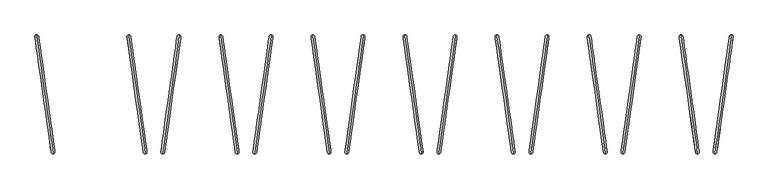
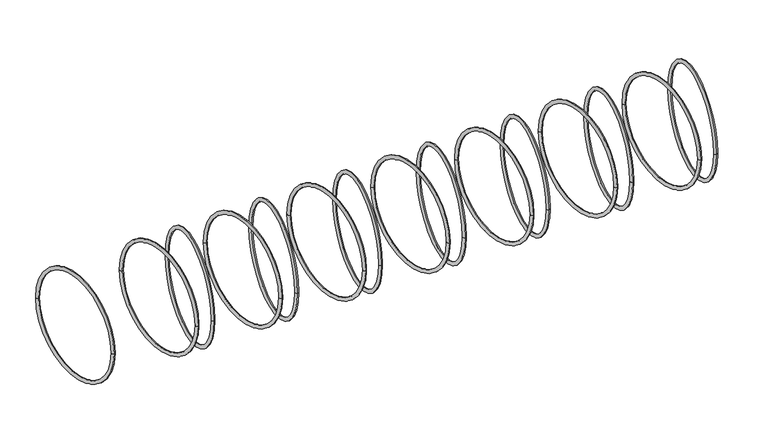
"""IFC4 building model written with IfcOpenShell, lengths in millimetres: geographic element geometry, NLRS_90_SI_WPB_fietsenrek staal_gen_bf : fietsenrek 5500mm 14 plaatsen."""

from ifc_helpers import new_model, si_unit, point, frame, origin, place, context, project, spatial, circle_curve, ellipse_curve, trimmed, source, transform, mapped, element, save
from ifc_brep_helpers import revolved_surface, advanced_brep


def geographic_element_fc57ddb0(model_context):
    return source(origin(), model_context, "Body", "AdvancedBrep", [
        advanced_brep(
        [(2160.5888305, 21.9255981, 304.7993564), (2162.7982034, 6.2050925, 304.7993564), (2089.8888952, 524.981777, 304.7993564), (2092.0982681, 509.2612714, 304.7993564)],
        [
            (0, 1, circle_curve(frame((2161.6935169, 14.0653453, 304.7993564), z_axis=(0.0, 0.0, 1.0), x_axis=(-0.1391731009600606, 0.990268068741571, 0.0)), 7.9375)),
            (1, 2, circle_curve(frame((2126.3435493, 265.5934347, 304.7993564), z_axis=(-0.990268068741571, -0.13917310096006058, 0.0), x_axis=(-0.13917310096006058, 0.990268068741571, 0.0)), 261.9375)),
            (2, 3, circle_curve(frame((2090.9935817, 517.1215242, 304.7993564), z_axis=(0.0, 0.0, 1.0), x_axis=(0.13917310096006055, -0.990268068741571, 0.0)), 7.9375)),
            (3, 0, circle_curve(frame((2126.3435493, 265.5934347, 304.7993564), z_axis=(0.990268068741571, 0.13917310096006058, 0.0), x_axis=(-0.13917310096006058, 0.990268068741571, 0.0)), 246.0625)),
            (1, 0, circle_curve(frame((2161.6935169, 14.0653453, 304.7993564), z_axis=(0.0, 0.0, 1.0), x_axis=(-0.1391731009600606, 0.990268068741571, 0.0)), 7.9375)),
            (3, 2, circle_curve(frame((2090.9935817, 517.1215242, 304.7993564), z_axis=(0.0, 0.0, 1.0), x_axis=(0.13917310096006055, -0.990268068741571, 0.0)), 7.9375)),
            (2, 1, circle_curve(frame((2126.3435493, 265.5934347, 304.7993564), z_axis=(-0.990268068741571, -0.13917310096006058, 0.0), x_axis=(0.13917310096006058, -0.990268068741571, 0.0)), 261.9375)),
            (0, 3, circle_curve(frame((2126.3435493, 265.5934347, 304.7993564), z_axis=(0.990268068741571, 0.13917310096006058, 0.0), x_axis=(0.13917310096006058, -0.990268068741571, 0.0)), 246.0625)),
        ],
        [
            revolved_surface(trimmed(ellipse_curve(frame((2090.9935817, 517.1215242, 304.7993564), z_axis=(0.0, 0.0, 1.0), x_axis=(0.13917310096006055, -0.990268068741571, 0.0)), 7.9375, 7.9375), [point((2089.8888952, 524.981777, 304.7993564))], [point((2092.0982681, 509.2612714, 304.7993564))], True, "CARTESIAN"), (2314.9896164, 292.1059105, 304.7993564), (-0.990268068741571, -0.13917310096006058, 0.0)),
            revolved_surface(trimmed(ellipse_curve(frame((2090.9935817, 517.1215242, 304.7993564), z_axis=(0.0, 0.0, 1.0), x_axis=(0.13917310096006055, -0.990268068741571, 0.0)), 7.9375, 7.9375), [point((2092.0982681, 509.2612714, 304.7993564))], [point((2089.8888952, 524.981777, 304.7993564))], True, "CARTESIAN"), (2314.9896164, 292.1059105, 304.7993564), (-0.990268068741571, -0.13917310096006058, 0.0)),
            revolved_surface(trimmed(ellipse_curve(frame((2161.6935169, 14.0653453, 304.7993564), z_axis=(0.0, 0.0, -1.0), x_axis=(-0.13917310096006055, 0.990268068741571, 0.0)), 7.9375, 7.9375), [point((2162.7982034, 6.2050925, 304.7993564))], [point((2160.5888305, 21.9255981, 304.7993564))], True, "CARTESIAN"), (2314.9896164, 292.1059105, 304.7993564), (-0.990268068741571, -0.13917310096006058, 0.0)),
            revolved_surface(trimmed(ellipse_curve(frame((2161.6935169, 14.0653453, 304.7993564), z_axis=(0.0, 0.0, -1.0), x_axis=(-0.13917310096006055, 0.990268068741571, 0.0)), 7.9375, 7.9375), [point((2160.5888305, 21.9255981, 304.7993564))], [point((2162.7982034, 6.2050925, 304.7993564))], True, "CARTESIAN"), (2314.9896164, 292.1059105, 304.7993564), (-0.990268068741571, -0.13917310096006058, 0.0)),
        ],
        [
            (0, [[1, 2, 3, 4]]),
            (1, [[5, -4, 6, -2]]),
            (2, [[-3, 7, -1, 8]]),
            (3, [[-6, -8, -5, -7]]),
        ],
    ),
        advanced_brep(
        [(2239.4111695, 21.9255981, 304.7993564), (2237.2017966, 6.2050925, 304.7993564), (2310.1111048, 524.981777, 304.7993564), (2307.9017319, 509.2612714, 304.7993564)],
        [
            (0, 1, circle_curve(frame((2238.3064831, 14.0653453, 304.7993564), z_axis=(0.0, 0.0, 1.0), x_axis=(0.13917310096005764, 0.9902680687415715, 0.0)), 7.9375)),
            (1, 2, circle_curve(frame((2273.6564507, 265.5934347, 304.7993564), z_axis=(-0.9902680687415715, 0.1391731009600577, 0.0), x_axis=(0.1391731009600577, 0.9902680687415715, 0.0)), 261.9375)),
            (2, 3, circle_curve(frame((2309.0064183, 517.1215242, 304.7993564), z_axis=(0.0, 0.0, 1.0), x_axis=(-0.13917310096005775, -0.9902680687415715, 0.0)), 7.9375)),
            (3, 0, circle_curve(frame((2273.6564507, 265.5934347, 304.7993564), z_axis=(0.9902680687415715, -0.1391731009600577, 0.0), x_axis=(0.1391731009600577, 0.9902680687415715, 0.0)), 246.0625)),
            (1, 0, circle_curve(frame((2238.3064831, 14.0653453, 304.7993564), z_axis=(0.0, 0.0, 1.0), x_axis=(0.13917310096005764, 0.9902680687415715, 0.0)), 7.9375)),
            (3, 2, circle_curve(frame((2309.0064183, 517.1215242, 304.7993564), z_axis=(0.0, 0.0, 1.0), x_axis=(-0.13917310096005775, -0.9902680687415715, 0.0)), 7.9375)),
            (2, 1, circle_curve(frame((2273.6564507, 265.5934347, 304.7993564), z_axis=(-0.9902680687415715, 0.1391731009600577, 0.0), x_axis=(-0.1391731009600577, -0.9902680687415715, 0.0)), 261.9375)),
            (0, 3, circle_curve(frame((2273.6564507, 265.5934347, 304.7993564), z_axis=(0.9902680687415715, -0.1391731009600577, 0.0), x_axis=(-0.1391731009600577, -0.9902680687415715, 0.0)), 246.0625)),
        ],
        [
            revolved_surface(trimmed(ellipse_curve(frame((2309.0064183, 517.1215242, 304.7993564), z_axis=(0.0, 0.0, 1.0), x_axis=(-0.13917310096005775, -0.9902680687415715, 0.0)), 7.9375, 7.9375), [point((2310.1111048, 524.981777, 304.7993564))], [point((2307.9017319, 509.2612714, 304.7993564))], True, "CARTESIAN"), (2085.0103836, 292.1059105, 304.7993564), (-0.9902680687415715, 0.1391731009600577, 0.0)),
            revolved_surface(trimmed(ellipse_curve(frame((2309.0064183, 517.1215242, 304.7993564), z_axis=(0.0, 0.0, 1.0), x_axis=(-0.13917310096005775, -0.9902680687415715, 0.0)), 7.9375, 7.9375), [point((2307.9017319, 509.2612714, 304.7993564))], [point((2310.1111048, 524.981777, 304.7993564))], True, "CARTESIAN"), (2085.0103836, 292.1059105, 304.7993564), (-0.9902680687415715, 0.1391731009600577, 0.0)),
            revolved_surface(trimmed(ellipse_curve(frame((2238.3064831, 14.0653453, 304.7993564), z_axis=(0.0, 0.0, -1.0), x_axis=(0.1391731009600577, 0.9902680687415715, 0.0)), 7.9375, 7.9375), [point((2237.2017966, 6.2050925, 304.7993564))], [point((2239.4111695, 21.9255981, 304.7993564))], True, "CARTESIAN"), (2085.0103836, 292.1059105, 304.7993564), (-0.9902680687415715, 0.1391731009600577, 0.0)),
            revolved_surface(trimmed(ellipse_curve(frame((2238.3064831, 14.0653453, 304.7993564), z_axis=(0.0, 0.0, -1.0), x_axis=(0.1391731009600577, 0.9902680687415715, 0.0)), 7.9375, 7.9375), [point((2239.4111695, 21.9255981, 304.7993564))], [point((2237.2017966, 6.2050925, 304.7993564))], True, "CARTESIAN"), (2085.0103836, 292.1059105, 304.7993564), (-0.9902680687415715, 0.1391731009600577, 0.0)),
        ],
        [
            (0, [[1, 2, 3, 4]]),
            (1, [[5, -4, 6, -2]]),
            (2, [[-3, 7, -1, 8]]),
            (3, [[-6, -8, -5, -7]]),
        ],
    ),
        advanced_brep(
        [(1760.5888305, 21.9255981, 304.7993564), (1762.7982034, 6.2050925, 304.7993564), (1689.8888952, 524.981777, 304.7993564), (1692.0982681, 509.2612714, 304.7993564)],
        [
            (0, 1, circle_curve(frame((1761.6935169, 14.0653453, 304.7993564), z_axis=(0.0, 0.0, 1.0), x_axis=(-0.1391731009600606, 0.990268068741571, 0.0)), 7.9375)),
            (1, 2, circle_curve(frame((1726.3435493, 265.5934347, 304.7993564), z_axis=(-0.990268068741571, -0.13917310096006058, 0.0), x_axis=(-0.13917310096006058, 0.990268068741571, 0.0)), 261.9375)),
            (2, 3, circle_curve(frame((1690.9935817, 517.1215242, 304.7993564), z_axis=(0.0, 0.0, 1.0), x_axis=(0.13917310096006055, -0.990268068741571, 0.0)), 7.9375)),
            (3, 0, circle_curve(frame((1726.3435493, 265.5934347, 304.7993564), z_axis=(0.990268068741571, 0.13917310096006058, 0.0), x_axis=(-0.13917310096006058, 0.990268068741571, 0.0)), 246.0625)),
            (1, 0, circle_curve(frame((1761.6935169, 14.0653453, 304.7993564), z_axis=(0.0, 0.0, 1.0), x_axis=(-0.1391731009600606, 0.990268068741571, 0.0)), 7.9375)),
            (3, 2, circle_curve(frame((1690.9935817, 517.1215242, 304.7993564), z_axis=(0.0, 0.0, 1.0), x_axis=(0.13917310096006055, -0.990268068741571, 0.0)), 7.9375)),
            (2, 1, circle_curve(frame((1726.3435493, 265.5934347, 304.7993564), z_axis=(-0.990268068741571, -0.13917310096006058, 0.0), x_axis=(0.13917310096006058, -0.990268068741571, 0.0)), 261.9375)),
            (0, 3, circle_curve(frame((1726.3435493, 265.5934347, 304.7993564), z_axis=(0.990268068741571, 0.13917310096006058, 0.0), x_axis=(0.13917310096006058, -0.990268068741571, 0.0)), 246.0625)),
        ],
        [
            revolved_surface(trimmed(ellipse_curve(frame((1690.9935817, 517.1215242, 304.7993564), z_axis=(0.0, 0.0, 1.0), x_axis=(0.13917310096006055, -0.990268068741571, 0.0)), 7.9375, 7.9375), [point((1689.8888952, 524.981777, 304.7993564))], [point((1692.0982681, 509.2612714, 304.7993564))], True, "CARTESIAN"), (1914.9896164, 292.1059105, 304.7993564), (-0.990268068741571, -0.13917310096006058, 0.0)),
            revolved_surface(trimmed(ellipse_curve(frame((1690.9935817, 517.1215242, 304.7993564), z_axis=(0.0, 0.0, 1.0), x_axis=(0.13917310096006055, -0.990268068741571, 0.0)), 7.9375, 7.9375), [point((1692.0982681, 509.2612714, 304.7993564))], [point((1689.8888952, 524.981777, 304.7993564))], True, "CARTESIAN"), (1914.9896164, 292.1059105, 304.7993564), (-0.990268068741571, -0.13917310096006058, 0.0)),
            revolved_surface(trimmed(ellipse_curve(frame((1761.6935169, 14.0653453, 304.7993564), z_axis=(0.0, 0.0, -1.0), x_axis=(-0.13917310096006055, 0.990268068741571, 0.0)), 7.9375, 7.9375), [point((1762.7982034, 6.2050925, 304.7993564))], [point((1760.5888305, 21.9255981, 304.7993564))], True, "CARTESIAN"), (1914.9896164, 292.1059105, 304.7993564), (-0.990268068741571, -0.13917310096006058, 0.0)),
            revolved_surface(trimmed(ellipse_curve(frame((1761.6935169, 14.0653453, 304.7993564), z_axis=(0.0, 0.0, -1.0), x_axis=(-0.13917310096006055, 0.990268068741571, 0.0)), 7.9375, 7.9375), [point((1760.5888305, 21.9255981, 304.7993564))], [point((1762.7982034, 6.2050925, 304.7993564))], True, "CARTESIAN"), (1914.9896164, 292.1059105, 304.7993564), (-0.990268068741571, -0.13917310096006058, 0.0)),
        ],
        [
            (0, [[1, 2, 3, 4]]),
            (1, [[5, -4, 6, -2]]),
            (2, [[-3, 7, -1, 8]]),
            (3, [[-6, -8, -5, -7]]),
        ],
    ),
        advanced_brep(
        [(1839.4111695, 21.9255981, 304.7993564), (1837.2017966, 6.2050925, 304.7993564), (1910.1111048, 524.981777, 304.7993564), (1907.9017319, 509.2612714, 304.7993564)],
        [
            (0, 1, circle_curve(frame((1838.3064831, 14.0653453, 304.7993564), z_axis=(0.0, 0.0, 1.0), x_axis=(0.13917310096005764, 0.9902680687415715, 0.0)), 7.9375)),
            (1, 2, circle_curve(frame((1873.6564507, 265.5934347, 304.7993564), z_axis=(-0.9902680687415715, 0.1391731009600577, 0.0), x_axis=(0.1391731009600577, 0.9902680687415715, 0.0)), 261.9375)),
            (2, 3, circle_curve(frame((1909.0064183, 517.1215242, 304.7993564), z_axis=(0.0, 0.0, 1.0), x_axis=(-0.13917310096005775, -0.9902680687415715, 0.0)), 7.9375)),
            (3, 0, circle_curve(frame((1873.6564507, 265.5934347, 304.7993564), z_axis=(0.9902680687415715, -0.1391731009600577, 0.0), x_axis=(0.1391731009600577, 0.9902680687415715, 0.0)), 246.0625)),
            (1, 0, circle_curve(frame((1838.3064831, 14.0653453, 304.7993564), z_axis=(0.0, 0.0, 1.0), x_axis=(0.13917310096005764, 0.9902680687415715, 0.0)), 7.9375)),
            (3, 2, circle_curve(frame((1909.0064183, 517.1215242, 304.7993564), z_axis=(0.0, 0.0, 1.0), x_axis=(-0.13917310096005775, -0.9902680687415715, 0.0)), 7.9375)),
            (2, 1, circle_curve(frame((1873.6564507, 265.5934347, 304.7993564), z_axis=(-0.9902680687415715, 0.1391731009600577, 0.0), x_axis=(-0.1391731009600577, -0.9902680687415715, 0.0)), 261.9375)),
            (0, 3, circle_curve(frame((1873.6564507, 265.5934347, 304.7993564), z_axis=(0.9902680687415715, -0.1391731009600577, 0.0), x_axis=(-0.1391731009600577, -0.9902680687415715, 0.0)), 246.0625)),
        ],
        [
            revolved_surface(trimmed(ellipse_curve(frame((1909.0064183, 517.1215242, 304.7993564), z_axis=(0.0, 0.0, 1.0), x_axis=(-0.13917310096005775, -0.9902680687415715, 0.0)), 7.9375, 7.9375), [point((1910.1111048, 524.981777, 304.7993564))], [point((1907.9017319, 509.2612714, 304.7993564))], True, "CARTESIAN"), (1685.0103836, 292.1059105, 304.7993564), (-0.9902680687415715, 0.1391731009600577, 0.0)),
            revolved_surface(trimmed(ellipse_curve(frame((1909.0064183, 517.1215242, 304.7993564), z_axis=(0.0, 0.0, 1.0), x_axis=(-0.13917310096005775, -0.9902680687415715, 0.0)), 7.9375, 7.9375), [point((1907.9017319, 509.2612714, 304.7993564))], [point((1910.1111048, 524.981777, 304.7993564))], True, "CARTESIAN"), (1685.0103836, 292.1059105, 304.7993564), (-0.9902680687415715, 0.1391731009600577, 0.0)),
            revolved_surface(trimmed(ellipse_curve(frame((1838.3064831, 14.0653453, 304.7993564), z_axis=(0.0, 0.0, -1.0), x_axis=(0.1391731009600577, 0.9902680687415715, 0.0)), 7.9375, 7.9375), [point((1837.2017966, 6.2050925, 304.7993564))], [point((1839.4111695, 21.9255981, 304.7993564))], True, "CARTESIAN"), (1685.0103836, 292.1059105, 304.7993564), (-0.9902680687415715, 0.1391731009600577, 0.0)),
            revolved_surface(trimmed(ellipse_curve(frame((1838.3064831, 14.0653453, 304.7993564), z_axis=(0.0, 0.0, -1.0), x_axis=(0.1391731009600577, 0.9902680687415715, 0.0)), 7.9375, 7.9375), [point((1839.4111695, 21.9255981, 304.7993564))], [point((1837.2017966, 6.2050925, 304.7993564))], True, "CARTESIAN"), (1685.0103836, 292.1059105, 304.7993564), (-0.9902680687415715, 0.1391731009600577, 0.0)),
        ],
        [
            (0, [[1, 2, 3, 4]]),
            (1, [[5, -4, 6, -2]]),
            (2, [[-3, 7, -1, 8]]),
            (3, [[-6, -8, -5, -7]]),
        ],
    ),
        advanced_brep(
        [(1360.5888305, 21.9255981, 304.7993564), (1362.7982034, 6.2050925, 304.7993564), (1289.8888952, 524.981777, 304.7993564), (1292.0982681, 509.2612714, 304.7993564)],
        [
            (0, 1, circle_curve(frame((1361.6935169, 14.0653453, 304.7993564), z_axis=(0.0, 0.0, 1.0), x_axis=(-0.1391731009600606, 0.990268068741571, 0.0)), 7.9375)),
            (1, 2, circle_curve(frame((1326.3435493, 265.5934347, 304.7993564), z_axis=(-0.990268068741571, -0.13917310096006058, 0.0), x_axis=(-0.13917310096006058, 0.990268068741571, 0.0)), 261.9375)),
            (2, 3, circle_curve(frame((1290.9935817, 517.1215242, 304.7993564), z_axis=(0.0, 0.0, 1.0), x_axis=(0.13917310096006055, -0.990268068741571, 0.0)), 7.9375)),
            (3, 0, circle_curve(frame((1326.3435493, 265.5934347, 304.7993564), z_axis=(0.990268068741571, 0.13917310096006058, 0.0), x_axis=(-0.13917310096006058, 0.990268068741571, 0.0)), 246.0625)),
            (1, 0, circle_curve(frame((1361.6935169, 14.0653453, 304.7993564), z_axis=(0.0, 0.0, 1.0), x_axis=(-0.1391731009600606, 0.990268068741571, 0.0)), 7.9375)),
            (3, 2, circle_curve(frame((1290.9935817, 517.1215242, 304.7993564), z_axis=(0.0, 0.0, 1.0), x_axis=(0.13917310096006055, -0.990268068741571, 0.0)), 7.9375)),
            (2, 1, circle_curve(frame((1326.3435493, 265.5934347, 304.7993564), z_axis=(-0.990268068741571, -0.13917310096006058, 0.0), x_axis=(0.13917310096006058, -0.990268068741571, 0.0)), 261.9375)),
            (0, 3, circle_curve(frame((1326.3435493, 265.5934347, 304.7993564), z_axis=(0.990268068741571, 0.13917310096006058, 0.0), x_axis=(0.13917310096006058, -0.990268068741571, 0.0)), 246.0625)),
        ],
        [
            revolved_surface(trimmed(ellipse_curve(frame((1290.9935817, 517.1215242, 304.7993564), z_axis=(0.0, 0.0, 1.0), x_axis=(0.13917310096006055, -0.990268068741571, 0.0)), 7.9375, 7.9375), [point((1289.8888952, 524.981777, 304.7993564))], [point((1292.0982681, 509.2612714, 304.7993564))], True, "CARTESIAN"), (1514.9896164, 292.1059105, 304.7993564), (-0.990268068741571, -0.13917310096006058, 0.0)),
            revolved_surface(trimmed(ellipse_curve(frame((1290.9935817, 517.1215242, 304.7993564), z_axis=(0.0, 0.0, 1.0), x_axis=(0.13917310096006055, -0.990268068741571, 0.0)), 7.9375, 7.9375), [point((1292.0982681, 509.2612714, 304.7993564))], [point((1289.8888952, 524.981777, 304.7993564))], True, "CARTESIAN"), (1514.9896164, 292.1059105, 304.7993564), (-0.990268068741571, -0.13917310096006058, 0.0)),
            revolved_surface(trimmed(ellipse_curve(frame((1361.6935169, 14.0653453, 304.7993564), z_axis=(0.0, 0.0, -1.0), x_axis=(-0.13917310096006055, 0.990268068741571, 0.0)), 7.9375, 7.9375), [point((1362.7982034, 6.2050925, 304.7993564))], [point((1360.5888305, 21.9255981, 304.7993564))], True, "CARTESIAN"), (1514.9896164, 292.1059105, 304.7993564), (-0.990268068741571, -0.13917310096006058, 0.0)),
            revolved_surface(trimmed(ellipse_curve(frame((1361.6935169, 14.0653453, 304.7993564), z_axis=(0.0, 0.0, -1.0), x_axis=(-0.13917310096006055, 0.990268068741571, 0.0)), 7.9375, 7.9375), [point((1360.5888305, 21.9255981, 304.7993564))], [point((1362.7982034, 6.2050925, 304.7993564))], True, "CARTESIAN"), (1514.9896164, 292.1059105, 304.7993564), (-0.990268068741571, -0.13917310096006058, 0.0)),
        ],
        [
            (0, [[1, 2, 3, 4]]),
            (1, [[5, -4, 6, -2]]),
            (2, [[-3, 7, -1, 8]]),
            (3, [[-6, -8, -5, -7]]),
        ],
    ),
        advanced_brep(
        [(1439.4111695, 21.9255981, 304.7993564), (1437.2017966, 6.2050925, 304.7993564), (1510.1111048, 524.981777, 304.7993564), (1507.9017319, 509.2612714, 304.7993564)],
        [
            (0, 1, circle_curve(frame((1438.3064831, 14.0653453, 304.7993564), z_axis=(0.0, 0.0, 1.0), x_axis=(0.13917310096005764, 0.9902680687415715, 0.0)), 7.9375)),
            (1, 2, circle_curve(frame((1473.6564507, 265.5934347, 304.7993564), z_axis=(-0.9902680687415715, 0.1391731009600577, 0.0), x_axis=(0.1391731009600577, 0.9902680687415715, 0.0)), 261.9375)),
            (2, 3, circle_curve(frame((1509.0064183, 517.1215242, 304.7993564), z_axis=(0.0, 0.0, 1.0), x_axis=(-0.13917310096005775, -0.9902680687415715, 0.0)), 7.9375)),
            (3, 0, circle_curve(frame((1473.6564507, 265.5934347, 304.7993564), z_axis=(0.9902680687415715, -0.1391731009600577, 0.0), x_axis=(0.1391731009600577, 0.9902680687415715, 0.0)), 246.0625)),
            (1, 0, circle_curve(frame((1438.3064831, 14.0653453, 304.7993564), z_axis=(0.0, 0.0, 1.0), x_axis=(0.13917310096005764, 0.9902680687415715, 0.0)), 7.9375)),
            (3, 2, circle_curve(frame((1509.0064183, 517.1215242, 304.7993564), z_axis=(0.0, 0.0, 1.0), x_axis=(-0.13917310096005775, -0.9902680687415715, 0.0)), 7.9375)),
            (2, 1, circle_curve(frame((1473.6564507, 265.5934347, 304.7993564), z_axis=(-0.9902680687415715, 0.1391731009600577, 0.0), x_axis=(-0.1391731009600577, -0.9902680687415715, 0.0)), 261.9375)),
            (0, 3, circle_curve(frame((1473.6564507, 265.5934347, 304.7993564), z_axis=(0.9902680687415715, -0.1391731009600577, 0.0), x_axis=(-0.1391731009600577, -0.9902680687415715, 0.0)), 246.0625)),
        ],
        [
            revolved_surface(trimmed(ellipse_curve(frame((1509.0064183, 517.1215242, 304.7993564), z_axis=(0.0, 0.0, 1.0), x_axis=(-0.13917310096005775, -0.9902680687415715, 0.0)), 7.9375, 7.9375), [point((1510.1111048, 524.981777, 304.7993564))], [point((1507.9017319, 509.2612714, 304.7993564))], True, "CARTESIAN"), (1285.0103836, 292.1059105, 304.7993564), (-0.9902680687415715, 0.1391731009600577, 0.0)),
            revolved_surface(trimmed(ellipse_curve(frame((1509.0064183, 517.1215242, 304.7993564), z_axis=(0.0, 0.0, 1.0), x_axis=(-0.13917310096005775, -0.9902680687415715, 0.0)), 7.9375, 7.9375), [point((1507.9017319, 509.2612714, 304.7993564))], [point((1510.1111048, 524.981777, 304.7993564))], True, "CARTESIAN"), (1285.0103836, 292.1059105, 304.7993564), (-0.9902680687415715, 0.1391731009600577, 0.0)),
            revolved_surface(trimmed(ellipse_curve(frame((1438.3064831, 14.0653453, 304.7993564), z_axis=(0.0, 0.0, -1.0), x_axis=(0.1391731009600577, 0.9902680687415715, 0.0)), 7.9375, 7.9375), [point((1437.2017966, 6.2050925, 304.7993564))], [point((1439.4111695, 21.9255981, 304.7993564))], True, "CARTESIAN"), (1285.0103836, 292.1059105, 304.7993564), (-0.9902680687415715, 0.1391731009600577, 0.0)),
            revolved_surface(trimmed(ellipse_curve(frame((1438.3064831, 14.0653453, 304.7993564), z_axis=(0.0, 0.0, -1.0), x_axis=(0.1391731009600577, 0.9902680687415715, 0.0)), 7.9375, 7.9375), [point((1439.4111695, 21.9255981, 304.7993564))], [point((1437.2017966, 6.2050925, 304.7993564))], True, "CARTESIAN"), (1285.0103836, 292.1059105, 304.7993564), (-0.9902680687415715, 0.1391731009600577, 0.0)),
        ],
        [
            (0, [[1, 2, 3, 4]]),
            (1, [[5, -4, 6, -2]]),
            (2, [[-3, 7, -1, 8]]),
            (3, [[-6, -8, -5, -7]]),
        ],
    ),
        advanced_brep(
        [(960.5888305, 21.9255981, 304.7993564), (962.7982034, 6.2050925, 304.7993564), (889.8888952, 524.981777, 304.7993564), (892.0982681, 509.2612714, 304.7993564)],
        [
            (0, 1, circle_curve(frame((961.6935169, 14.0653453, 304.7993564), z_axis=(0.0, 0.0, 1.0), x_axis=(-0.1391731009600606, 0.990268068741571, 0.0)), 7.9375)),
            (1, 2, circle_curve(frame((926.3435493, 265.5934347, 304.7993564), z_axis=(-0.990268068741571, -0.13917310096006058, 0.0), x_axis=(-0.13917310096006058, 0.990268068741571, 0.0)), 261.9375)),
            (2, 3, circle_curve(frame((890.9935817, 517.1215242, 304.7993564), z_axis=(0.0, 0.0, 1.0), x_axis=(0.13917310096006055, -0.990268068741571, 0.0)), 7.9375)),
            (3, 0, circle_curve(frame((926.3435493, 265.5934347, 304.7993564), z_axis=(0.990268068741571, 0.13917310096006058, 0.0), x_axis=(-0.13917310096006058, 0.990268068741571, 0.0)), 246.0625)),
            (1, 0, circle_curve(frame((961.6935169, 14.0653453, 304.7993564), z_axis=(0.0, 0.0, 1.0), x_axis=(-0.1391731009600606, 0.990268068741571, 0.0)), 7.9375)),
            (3, 2, circle_curve(frame((890.9935817, 517.1215242, 304.7993564), z_axis=(0.0, 0.0, 1.0), x_axis=(0.13917310096006055, -0.990268068741571, 0.0)), 7.9375)),
            (2, 1, circle_curve(frame((926.3435493, 265.5934347, 304.7993564), z_axis=(-0.990268068741571, -0.13917310096006058, 0.0), x_axis=(0.13917310096006058, -0.990268068741571, 0.0)), 261.9375)),
            (0, 3, circle_curve(frame((926.3435493, 265.5934347, 304.7993564), z_axis=(0.990268068741571, 0.13917310096006058, 0.0), x_axis=(0.13917310096006058, -0.990268068741571, 0.0)), 246.0625)),
        ],
        [
            revolved_surface(trimmed(ellipse_curve(frame((890.9935817, 517.1215242, 304.7993564), z_axis=(0.0, 0.0, 1.0), x_axis=(0.13917310096006055, -0.990268068741571, 0.0)), 7.9375, 7.9375), [point((889.8888952, 524.981777, 304.7993564))], [point((892.0982681, 509.2612714, 304.7993564))], True, "CARTESIAN"), (1114.9896164, 292.1059105, 304.7993564), (-0.990268068741571, -0.13917310096006058, 0.0)),
            revolved_surface(trimmed(ellipse_curve(frame((890.9935817, 517.1215242, 304.7993564), z_axis=(0.0, 0.0, 1.0), x_axis=(0.13917310096006055, -0.990268068741571, 0.0)), 7.9375, 7.9375), [point((892.0982681, 509.2612714, 304.7993564))], [point((889.8888952, 524.981777, 304.7993564))], True, "CARTESIAN"), (1114.9896164, 292.1059105, 304.7993564), (-0.990268068741571, -0.13917310096006058, 0.0)),
            revolved_surface(trimmed(ellipse_curve(frame((961.6935169, 14.0653453, 304.7993564), z_axis=(0.0, 0.0, -1.0), x_axis=(-0.13917310096006055, 0.990268068741571, 0.0)), 7.9375, 7.9375), [point((962.7982034, 6.2050925, 304.7993564))], [point((960.5888305, 21.9255981, 304.7993564))], True, "CARTESIAN"), (1114.9896164, 292.1059105, 304.7993564), (-0.990268068741571, -0.13917310096006058, 0.0)),
            revolved_surface(trimmed(ellipse_curve(frame((961.6935169, 14.0653453, 304.7993564), z_axis=(0.0, 0.0, -1.0), x_axis=(-0.13917310096006055, 0.990268068741571, 0.0)), 7.9375, 7.9375), [point((960.5888305, 21.9255981, 304.7993564))], [point((962.7982034, 6.2050925, 304.7993564))], True, "CARTESIAN"), (1114.9896164, 292.1059105, 304.7993564), (-0.990268068741571, -0.13917310096006058, 0.0)),
        ],
        [
            (0, [[1, 2, 3, 4]]),
            (1, [[5, -4, 6, -2]]),
            (2, [[-3, 7, -1, 8]]),
            (3, [[-6, -8, -5, -7]]),
        ],
    ),
        advanced_brep(
        [(1039.4111695, 21.9255981, 304.7993564), (1037.2017966, 6.2050925, 304.7993564), (1110.1111048, 524.981777, 304.7993564), (1107.9017319, 509.2612714, 304.7993564)],
        [
            (0, 1, circle_curve(frame((1038.3064831, 14.0653453, 304.7993564), z_axis=(0.0, 0.0, 1.0), x_axis=(0.13917310096005764, 0.9902680687415715, 0.0)), 7.9375)),
            (1, 2, circle_curve(frame((1073.6564507, 265.5934347, 304.7993564), z_axis=(-0.9902680687415715, 0.1391731009600577, 0.0), x_axis=(0.1391731009600577, 0.9902680687415715, 0.0)), 261.9375)),
            (2, 3, circle_curve(frame((1109.0064183, 517.1215242, 304.7993564), z_axis=(0.0, 0.0, 1.0), x_axis=(-0.13917310096005775, -0.9902680687415715, 0.0)), 7.9375)),
            (3, 0, circle_curve(frame((1073.6564507, 265.5934347, 304.7993564), z_axis=(0.9902680687415715, -0.1391731009600577, 0.0), x_axis=(0.1391731009600577, 0.9902680687415715, 0.0)), 246.0625)),
            (1, 0, circle_curve(frame((1038.3064831, 14.0653453, 304.7993564), z_axis=(0.0, 0.0, 1.0), x_axis=(0.13917310096005764, 0.9902680687415715, 0.0)), 7.9375)),
            (3, 2, circle_curve(frame((1109.0064183, 517.1215242, 304.7993564), z_axis=(0.0, 0.0, 1.0), x_axis=(-0.13917310096005775, -0.9902680687415715, 0.0)), 7.9375)),
            (2, 1, circle_curve(frame((1073.6564507, 265.5934347, 304.7993564), z_axis=(-0.9902680687415715, 0.1391731009600577, 0.0), x_axis=(-0.1391731009600577, -0.9902680687415715, 0.0)), 261.9375)),
            (0, 3, circle_curve(frame((1073.6564507, 265.5934347, 304.7993564), z_axis=(0.9902680687415715, -0.1391731009600577, 0.0), x_axis=(-0.1391731009600577, -0.9902680687415715, 0.0)), 246.0625)),
        ],
        [
            revolved_surface(trimmed(ellipse_curve(frame((1109.0064183, 517.1215242, 304.7993564), z_axis=(0.0, 0.0, 1.0), x_axis=(-0.13917310096005775, -0.9902680687415715, 0.0)), 7.9375, 7.9375), [point((1110.1111048, 524.981777, 304.7993564))], [point((1107.9017319, 509.2612714, 304.7993564))], True, "CARTESIAN"), (885.0103836, 292.1059105, 304.7993564), (-0.9902680687415715, 0.1391731009600577, 0.0)),
            revolved_surface(trimmed(ellipse_curve(frame((1109.0064183, 517.1215242, 304.7993564), z_axis=(0.0, 0.0, 1.0), x_axis=(-0.13917310096005775, -0.9902680687415715, 0.0)), 7.9375, 7.9375), [point((1107.9017319, 509.2612714, 304.7993564))], [point((1110.1111048, 524.981777, 304.7993564))], True, "CARTESIAN"), (885.0103836, 292.1059105, 304.7993564), (-0.9902680687415715, 0.1391731009600577, 0.0)),
            revolved_surface(trimmed(ellipse_curve(frame((1038.3064831, 14.0653453, 304.7993564), z_axis=(0.0, 0.0, -1.0), x_axis=(0.1391731009600577, 0.9902680687415715, 0.0)), 7.9375, 7.9375), [point((1037.2017966, 6.2050925, 304.7993564))], [point((1039.4111695, 21.9255981, 304.7993564))], True, "CARTESIAN"), (885.0103836, 292.1059105, 304.7993564), (-0.9902680687415715, 0.1391731009600577, 0.0)),
            revolved_surface(trimmed(ellipse_curve(frame((1038.3064831, 14.0653453, 304.7993564), z_axis=(0.0, 0.0, -1.0), x_axis=(0.1391731009600577, 0.9902680687415715, 0.0)), 7.9375, 7.9375), [point((1039.4111695, 21.9255981, 304.7993564))], [point((1037.2017966, 6.2050925, 304.7993564))], True, "CARTESIAN"), (885.0103836, 292.1059105, 304.7993564), (-0.9902680687415715, 0.1391731009600577, 0.0)),
        ],
        [
            (0, [[1, 2, 3, 4]]),
            (1, [[5, -4, 6, -2]]),
            (2, [[-3, 7, -1, 8]]),
            (3, [[-6, -8, -5, -7]]),
        ],
    ),
        advanced_brep(
        [(560.5888305, 21.9255981, 304.7993564), (562.7982034, 6.2050925, 304.7993564), (489.8888952, 524.981777, 304.7993564), (492.0982681, 509.2612714, 304.7993564)],
        [
            (0, 1, circle_curve(frame((561.6935169, 14.0653453, 304.7993564), z_axis=(0.0, 0.0, 1.0), x_axis=(-0.1391731009600606, 0.990268068741571, 0.0)), 7.9375)),
            (1, 2, circle_curve(frame((526.3435493, 265.5934347, 304.7993564), z_axis=(-0.990268068741571, -0.13917310096006058, 0.0), x_axis=(-0.13917310096006058, 0.990268068741571, 0.0)), 261.9375)),
            (2, 3, circle_curve(frame((490.9935817, 517.1215242, 304.7993564), z_axis=(0.0, 0.0, 1.0), x_axis=(0.13917310096006055, -0.990268068741571, 0.0)), 7.9375)),
            (3, 0, circle_curve(frame((526.3435493, 265.5934347, 304.7993564), z_axis=(0.990268068741571, 0.13917310096006058, 0.0), x_axis=(-0.13917310096006058, 0.990268068741571, 0.0)), 246.0625)),
            (1, 0, circle_curve(frame((561.6935169, 14.0653453, 304.7993564), z_axis=(0.0, 0.0, 1.0), x_axis=(-0.1391731009600606, 0.990268068741571, 0.0)), 7.9375)),
            (3, 2, circle_curve(frame((490.9935817, 517.1215242, 304.7993564), z_axis=(0.0, 0.0, 1.0), x_axis=(0.13917310096006055, -0.990268068741571, 0.0)), 7.9375)),
            (2, 1, circle_curve(frame((526.3435493, 265.5934347, 304.7993564), z_axis=(-0.990268068741571, -0.13917310096006058, 0.0), x_axis=(0.13917310096006058, -0.990268068741571, 0.0)), 261.9375)),
            (0, 3, circle_curve(frame((526.3435493, 265.5934347, 304.7993564), z_axis=(0.990268068741571, 0.13917310096006058, 0.0), x_axis=(0.13917310096006058, -0.990268068741571, 0.0)), 246.0625)),
        ],
        [
            revolved_surface(trimmed(ellipse_curve(frame((490.9935817, 517.1215242, 304.7993564), z_axis=(0.0, 0.0, 1.0), x_axis=(0.13917310096006055, -0.990268068741571, 0.0)), 7.9375, 7.9375), [point((489.8888952, 524.981777, 304.7993564))], [point((492.0982681, 509.2612714, 304.7993564))], True, "CARTESIAN"), (714.9896164, 292.1059105, 304.7993564), (-0.990268068741571, -0.13917310096006058, 0.0)),
            revolved_surface(trimmed(ellipse_curve(frame((490.9935817, 517.1215242, 304.7993564), z_axis=(0.0, 0.0, 1.0), x_axis=(0.13917310096006055, -0.990268068741571, 0.0)), 7.9375, 7.9375), [point((492.0982681, 509.2612714, 304.7993564))], [point((489.8888952, 524.981777, 304.7993564))], True, "CARTESIAN"), (714.9896164, 292.1059105, 304.7993564), (-0.990268068741571, -0.13917310096006058, 0.0)),
            revolved_surface(trimmed(ellipse_curve(frame((561.6935169, 14.0653453, 304.7993564), z_axis=(0.0, 0.0, -1.0), x_axis=(-0.13917310096006055, 0.990268068741571, 0.0)), 7.9375, 7.9375), [point((562.7982034, 6.2050925, 304.7993564))], [point((560.5888305, 21.9255981, 304.7993564))], True, "CARTESIAN"), (714.9896164, 292.1059105, 304.7993564), (-0.990268068741571, -0.13917310096006058, 0.0)),
            revolved_surface(trimmed(ellipse_curve(frame((561.6935169, 14.0653453, 304.7993564), z_axis=(0.0, 0.0, -1.0), x_axis=(-0.13917310096006055, 0.990268068741571, 0.0)), 7.9375, 7.9375), [point((560.5888305, 21.9255981, 304.7993564))], [point((562.7982034, 6.2050925, 304.7993564))], True, "CARTESIAN"), (714.9896164, 292.1059105, 304.7993564), (-0.990268068741571, -0.13917310096006058, 0.0)),
        ],
        [
            (0, [[1, 2, 3, 4]]),
            (1, [[5, -4, 6, -2]]),
            (2, [[-3, 7, -1, 8]]),
            (3, [[-6, -8, -5, -7]]),
        ],
    ),
        advanced_brep(
        [(639.4111695, 21.9255981, 304.7993564), (637.2017966, 6.2050925, 304.7993564), (710.1111048, 524.981777, 304.7993564), (707.9017319, 509.2612714, 304.7993564)],
        [
            (0, 1, circle_curve(frame((638.3064831, 14.0653453, 304.7993564), z_axis=(0.0, 0.0, 1.0), x_axis=(0.13917310096005764, 0.9902680687415715, 0.0)), 7.9375)),
            (1, 2, circle_curve(frame((673.6564507, 265.5934347, 304.7993564), z_axis=(-0.9902680687415715, 0.1391731009600577, 0.0), x_axis=(0.1391731009600577, 0.9902680687415715, 0.0)), 261.9375)),
            (2, 3, circle_curve(frame((709.0064183, 517.1215242, 304.7993564), z_axis=(0.0, 0.0, 1.0), x_axis=(-0.13917310096005775, -0.9902680687415715, 0.0)), 7.9375)),
            (3, 0, circle_curve(frame((673.6564507, 265.5934347, 304.7993564), z_axis=(0.9902680687415715, -0.1391731009600577, 0.0), x_axis=(0.1391731009600577, 0.9902680687415715, 0.0)), 246.0625)),
            (1, 0, circle_curve(frame((638.3064831, 14.0653453, 304.7993564), z_axis=(0.0, 0.0, 1.0), x_axis=(0.13917310096005764, 0.9902680687415715, 0.0)), 7.9375)),
            (3, 2, circle_curve(frame((709.0064183, 517.1215242, 304.7993564), z_axis=(0.0, 0.0, 1.0), x_axis=(-0.13917310096005775, -0.9902680687415715, 0.0)), 7.9375)),
            (2, 1, circle_curve(frame((673.6564507, 265.5934347, 304.7993564), z_axis=(-0.9902680687415715, 0.1391731009600577, 0.0), x_axis=(-0.1391731009600577, -0.9902680687415715, 0.0)), 261.9375)),
            (0, 3, circle_curve(frame((673.6564507, 265.5934347, 304.7993564), z_axis=(0.9902680687415715, -0.1391731009600577, 0.0), x_axis=(-0.1391731009600577, -0.9902680687415715, 0.0)), 246.0625)),
        ],
        [
            revolved_surface(trimmed(ellipse_curve(frame((709.0064183, 517.1215242, 304.7993564), z_axis=(0.0, 0.0, 1.0), x_axis=(-0.13917310096005775, -0.9902680687415715, 0.0)), 7.9375, 7.9375), [point((710.1111048, 524.981777, 304.7993564))], [point((707.9017319, 509.2612714, 304.7993564))], True, "CARTESIAN"), (485.0103836, 292.1059105, 304.7993564), (-0.9902680687415715, 0.1391731009600577, 0.0)),
            revolved_surface(trimmed(ellipse_curve(frame((709.0064183, 517.1215242, 304.7993564), z_axis=(0.0, 0.0, 1.0), x_axis=(-0.13917310096005775, -0.9902680687415715, 0.0)), 7.9375, 7.9375), [point((707.9017319, 509.2612714, 304.7993564))], [point((710.1111048, 524.981777, 304.7993564))], True, "CARTESIAN"), (485.0103836, 292.1059105, 304.7993564), (-0.9902680687415715, 0.1391731009600577, 0.0)),
            revolved_surface(trimmed(ellipse_curve(frame((638.3064831, 14.0653453, 304.7993564), z_axis=(0.0, 0.0, -1.0), x_axis=(0.1391731009600577, 0.9902680687415715, 0.0)), 7.9375, 7.9375), [point((637.2017966, 6.2050925, 304.7993564))], [point((639.4111695, 21.9255981, 304.7993564))], True, "CARTESIAN"), (485.0103836, 292.1059105, 304.7993564), (-0.9902680687415715, 0.1391731009600577, 0.0)),
            revolved_surface(trimmed(ellipse_curve(frame((638.3064831, 14.0653453, 304.7993564), z_axis=(0.0, 0.0, -1.0), x_axis=(0.1391731009600577, 0.9902680687415715, 0.0)), 7.9375, 7.9375), [point((639.4111695, 21.9255981, 304.7993564))], [point((637.2017966, 6.2050925, 304.7993564))], True, "CARTESIAN"), (485.0103836, 292.1059105, 304.7993564), (-0.9902680687415715, 0.1391731009600577, 0.0)),
        ],
        [
            (0, [[1, 2, 3, 4]]),
            (1, [[5, -4, 6, -2]]),
            (2, [[-3, 7, -1, 8]]),
            (3, [[-6, -8, -5, -7]]),
        ],
    ),
        advanced_brep(
        [(160.5888305, 21.9255981, 304.7993564), (162.7982034, 6.2050925, 304.7993564), (89.8888952, 524.981777, 304.7993564), (92.0982681, 509.2612714, 304.7993564)],
        [
            (0, 1, circle_curve(frame((161.6935169, 14.0653453, 304.7993564), z_axis=(0.0, 0.0, 1.0), x_axis=(-0.1391731009600606, 0.990268068741571, 0.0)), 7.9375)),
            (1, 2, circle_curve(frame((126.3435493, 265.5934347, 304.7993564), z_axis=(-0.990268068741571, -0.13917310096006058, 0.0), x_axis=(-0.13917310096006058, 0.990268068741571, 0.0)), 261.9375)),
            (2, 3, circle_curve(frame((90.9935817, 517.1215242, 304.7993564), z_axis=(0.0, 0.0, 1.0), x_axis=(0.13917310096006055, -0.990268068741571, 0.0)), 7.9375)),
            (3, 0, circle_curve(frame((126.3435493, 265.5934347, 304.7993564), z_axis=(0.990268068741571, 0.13917310096006058, 0.0), x_axis=(-0.13917310096006058, 0.990268068741571, 0.0)), 246.0625)),
            (1, 0, circle_curve(frame((161.6935169, 14.0653453, 304.7993564), z_axis=(0.0, 0.0, 1.0), x_axis=(-0.1391731009600606, 0.990268068741571, 0.0)), 7.9375)),
            (3, 2, circle_curve(frame((90.9935817, 517.1215242, 304.7993564), z_axis=(0.0, 0.0, 1.0), x_axis=(0.13917310096006055, -0.990268068741571, 0.0)), 7.9375)),
            (2, 1, circle_curve(frame((126.3435493, 265.5934347, 304.7993564), z_axis=(-0.990268068741571, -0.13917310096006058, 0.0), x_axis=(0.13917310096006058, -0.990268068741571, 0.0)), 261.9375)),
            (0, 3, circle_curve(frame((126.3435493, 265.5934347, 304.7993564), z_axis=(0.990268068741571, 0.13917310096006058, 0.0), x_axis=(0.13917310096006058, -0.990268068741571, 0.0)), 246.0625)),
        ],
        [
            revolved_surface(trimmed(ellipse_curve(frame((90.9935817, 517.1215242, 304.7993564), z_axis=(0.0, 0.0, 1.0), x_axis=(0.13917310096006055, -0.990268068741571, 0.0)), 7.9375, 7.9375), [point((89.8888952, 524.981777, 304.7993564))], [point((92.0982681, 509.2612714, 304.7993564))], True, "CARTESIAN"), (314.9896164, 292.1059105, 304.7993564), (-0.990268068741571, -0.13917310096006058, 0.0)),
            revolved_surface(trimmed(ellipse_curve(frame((90.9935817, 517.1215242, 304.7993564), z_axis=(0.0, 0.0, 1.0), x_axis=(0.13917310096006055, -0.990268068741571, 0.0)), 7.9375, 7.9375), [point((92.0982681, 509.2612714, 304.7993564))], [point((89.8888952, 524.981777, 304.7993564))], True, "CARTESIAN"), (314.9896164, 292.1059105, 304.7993564), (-0.990268068741571, -0.13917310096006058, 0.0)),
            revolved_surface(trimmed(ellipse_curve(frame((161.6935169, 14.0653453, 304.7993564), z_axis=(0.0, 0.0, -1.0), x_axis=(-0.13917310096006055, 0.990268068741571, 0.0)), 7.9375, 7.9375), [point((162.7982034, 6.2050925, 304.7993564))], [point((160.5888305, 21.9255981, 304.7993564))], True, "CARTESIAN"), (314.9896164, 292.1059105, 304.7993564), (-0.990268068741571, -0.13917310096006058, 0.0)),
            revolved_surface(trimmed(ellipse_curve(frame((161.6935169, 14.0653453, 304.7993564), z_axis=(0.0, 0.0, -1.0), x_axis=(-0.13917310096006055, 0.990268068741571, 0.0)), 7.9375, 7.9375), [point((160.5888305, 21.9255981, 304.7993564))], [point((162.7982034, 6.2050925, 304.7993564))], True, "CARTESIAN"), (314.9896164, 292.1059105, 304.7993564), (-0.990268068741571, -0.13917310096006058, 0.0)),
        ],
        [
            (0, [[1, 2, 3, 4]]),
            (1, [[5, -4, 6, -2]]),
            (2, [[-3, 7, -1, 8]]),
            (3, [[-6, -8, -5, -7]]),
        ],
    ),
        advanced_brep(
        [(239.4111695, 21.9255981, 304.7993564), (237.2017966, 6.2050925, 304.7993564), (310.1111048, 524.981777, 304.7993564), (307.9017319, 509.2612714, 304.7993564)],
        [
            (0, 1, circle_curve(frame((238.3064831, 14.0653453, 304.7993564), z_axis=(0.0, 0.0, 1.0), x_axis=(0.13917310096005764, 0.9902680687415715, 0.0)), 7.9375)),
            (1, 2, circle_curve(frame((273.6564507, 265.5934347, 304.7993564), z_axis=(-0.9902680687415715, 0.1391731009600577, 0.0), x_axis=(0.1391731009600577, 0.9902680687415715, 0.0)), 261.9375)),
            (2, 3, circle_curve(frame((309.0064183, 517.1215242, 304.7993564), z_axis=(0.0, 0.0, 1.0), x_axis=(-0.13917310096005775, -0.9902680687415715, 0.0)), 7.9375)),
            (3, 0, circle_curve(frame((273.6564507, 265.5934347, 304.7993564), z_axis=(0.9902680687415715, -0.1391731009600577, 0.0), x_axis=(0.1391731009600577, 0.9902680687415715, 0.0)), 246.0625)),
            (1, 0, circle_curve(frame((238.3064831, 14.0653453, 304.7993564), z_axis=(0.0, 0.0, 1.0), x_axis=(0.13917310096005764, 0.9902680687415715, 0.0)), 7.9375)),
            (3, 2, circle_curve(frame((309.0064183, 517.1215242, 304.7993564), z_axis=(0.0, 0.0, 1.0), x_axis=(-0.13917310096005775, -0.9902680687415715, 0.0)), 7.9375)),
            (2, 1, circle_curve(frame((273.6564507, 265.5934347, 304.7993564), z_axis=(-0.9902680687415715, 0.1391731009600577, 0.0), x_axis=(-0.1391731009600577, -0.9902680687415715, 0.0)), 261.9375)),
            (0, 3, circle_curve(frame((273.6564507, 265.5934347, 304.7993564), z_axis=(0.9902680687415715, -0.1391731009600577, 0.0), x_axis=(-0.1391731009600577, -0.9902680687415715, 0.0)), 246.0625)),
        ],
        [
            revolved_surface(trimmed(ellipse_curve(frame((309.0064183, 517.1215242, 304.7993564), z_axis=(0.0, 0.0, 1.0), x_axis=(-0.13917310096005775, -0.9902680687415715, 0.0)), 7.9375, 7.9375), [point((310.1111048, 524.981777, 304.7993564))], [point((307.9017319, 509.2612714, 304.7993564))], True, "CARTESIAN"), (85.0103836, 292.1059105, 304.7993564), (-0.9902680687415715, 0.1391731009600577, 0.0)),
            revolved_surface(trimmed(ellipse_curve(frame((309.0064183, 517.1215242, 304.7993564), z_axis=(0.0, 0.0, 1.0), x_axis=(-0.13917310096005775, -0.9902680687415715, 0.0)), 7.9375, 7.9375), [point((307.9017319, 509.2612714, 304.7993564))], [point((310.1111048, 524.981777, 304.7993564))], True, "CARTESIAN"), (85.0103836, 292.1059105, 304.7993564), (-0.9902680687415715, 0.1391731009600577, 0.0)),
            revolved_surface(trimmed(ellipse_curve(frame((238.3064831, 14.0653453, 304.7993564), z_axis=(0.0, 0.0, -1.0), x_axis=(0.1391731009600577, 0.9902680687415715, 0.0)), 7.9375, 7.9375), [point((237.2017966, 6.2050925, 304.7993564))], [point((239.4111695, 21.9255981, 304.7993564))], True, "CARTESIAN"), (85.0103836, 292.1059105, 304.7993564), (-0.9902680687415715, 0.1391731009600577, 0.0)),
            revolved_surface(trimmed(ellipse_curve(frame((238.3064831, 14.0653453, 304.7993564), z_axis=(0.0, 0.0, -1.0), x_axis=(0.1391731009600577, 0.9902680687415715, 0.0)), 7.9375, 7.9375), [point((239.4111695, 21.9255981, 304.7993564))], [point((237.2017966, 6.2050925, 304.7993564))], True, "CARTESIAN"), (85.0103836, 292.1059105, 304.7993564), (-0.9902680687415715, 0.1391731009600577, 0.0)),
        ],
        [
            (0, [[1, 2, 3, 4]]),
            (1, [[5, -4, 6, -2]]),
            (2, [[-3, 7, -1, 8]]),
            (3, [[-6, -8, -5, -7]]),
        ],
    ),
        advanced_brep(
        [(-239.4111695, 21.9255981, 304.7993564), (-237.2017966, 6.2050925, 304.7993564), (-310.1111048, 524.981777, 304.7993564), (-307.9017319, 509.2612714, 304.7993564)],
        [
            (0, 1, circle_curve(frame((-238.3064831, 14.0653453, 304.7993564), z_axis=(0.0, 0.0, 1.0), x_axis=(-0.1391731009600606, 0.990268068741571, 0.0)), 7.9375)),
            (1, 2, circle_curve(frame((-273.6564507, 265.5934347, 304.7993564), z_axis=(-0.990268068741571, -0.13917310096006058, 0.0), x_axis=(-0.13917310096006058, 0.990268068741571, 0.0)), 261.9375)),
            (2, 3, circle_curve(frame((-309.0064183, 517.1215242, 304.7993564), z_axis=(0.0, 0.0, 1.0), x_axis=(0.13917310096006055, -0.990268068741571, 0.0)), 7.9375)),
            (3, 0, circle_curve(frame((-273.6564507, 265.5934347, 304.7993564), z_axis=(0.990268068741571, 0.13917310096006058, 0.0), x_axis=(-0.13917310096006058, 0.990268068741571, 0.0)), 246.0625)),
            (1, 0, circle_curve(frame((-238.3064831, 14.0653453, 304.7993564), z_axis=(0.0, 0.0, 1.0), x_axis=(-0.1391731009600606, 0.990268068741571, 0.0)), 7.9375)),
            (3, 2, circle_curve(frame((-309.0064183, 517.1215242, 304.7993564), z_axis=(0.0, 0.0, 1.0), x_axis=(0.13917310096006055, -0.990268068741571, 0.0)), 7.9375)),
            (2, 1, circle_curve(frame((-273.6564507, 265.5934347, 304.7993564), z_axis=(-0.990268068741571, -0.13917310096006058, 0.0), x_axis=(0.13917310096006058, -0.990268068741571, 0.0)), 261.9375)),
            (0, 3, circle_curve(frame((-273.6564507, 265.5934347, 304.7993564), z_axis=(0.990268068741571, 0.13917310096006058, 0.0), x_axis=(0.13917310096006058, -0.990268068741571, 0.0)), 246.0625)),
        ],
        [
            revolved_surface(trimmed(ellipse_curve(frame((-309.0064183, 517.1215242, 304.7993564), z_axis=(0.0, 0.0, 1.0), x_axis=(0.13917310096006055, -0.990268068741571, 0.0)), 7.9375, 7.9375), [point((-310.1111048, 524.981777, 304.7993564))], [point((-307.9017319, 509.2612714, 304.7993564))], True, "CARTESIAN"), (-85.0103836, 292.1059105, 304.7993564), (-0.990268068741571, -0.13917310096006058, 0.0)),
            revolved_surface(trimmed(ellipse_curve(frame((-309.0064183, 517.1215242, 304.7993564), z_axis=(0.0, 0.0, 1.0), x_axis=(0.13917310096006055, -0.990268068741571, 0.0)), 7.9375, 7.9375), [point((-307.9017319, 509.2612714, 304.7993564))], [point((-310.1111048, 524.981777, 304.7993564))], True, "CARTESIAN"), (-85.0103836, 292.1059105, 304.7993564), (-0.990268068741571, -0.13917310096006058, 0.0)),
            revolved_surface(trimmed(ellipse_curve(frame((-238.3064831, 14.0653453, 304.7993564), z_axis=(0.0, 0.0, -1.0), x_axis=(-0.13917310096006055, 0.990268068741571, 0.0)), 7.9375, 7.9375), [point((-237.2017966, 6.2050925, 304.7993564))], [point((-239.4111695, 21.9255981, 304.7993564))], True, "CARTESIAN"), (-85.0103836, 292.1059105, 304.7993564), (-0.990268068741571, -0.13917310096006058, 0.0)),
            revolved_surface(trimmed(ellipse_curve(frame((-238.3064831, 14.0653453, 304.7993564), z_axis=(0.0, 0.0, -1.0), x_axis=(-0.13917310096006055, 0.990268068741571, 0.0)), 7.9375, 7.9375), [point((-239.4111695, 21.9255981, 304.7993564))], [point((-237.2017966, 6.2050925, 304.7993564))], True, "CARTESIAN"), (-85.0103836, 292.1059105, 304.7993564), (-0.990268068741571, -0.13917310096006058, 0.0)),
        ],
        [
            (0, [[1, 2, 3, 4]]),
            (1, [[5, -4, 6, -2]]),
            (2, [[-3, 7, -1, 8]]),
            (3, [[-6, -8, -5, -7]]),
        ],
    ),
        advanced_brep(
        [(-160.5888305, 21.9255981, 304.7993564), (-162.7982034, 6.2050925, 304.7993564), (-89.8888952, 524.981777, 304.7993564), (-92.0982681, 509.2612714, 304.7993564)],
        [
            (0, 1, circle_curve(frame((-161.6935169, 14.0653453, 304.7993564), z_axis=(0.0, 0.0, 1.0), x_axis=(0.13917310096005764, 0.9902680687415715, 0.0)), 7.9375)),
            (1, 2, circle_curve(frame((-126.3435493, 265.5934347, 304.7993564), z_axis=(-0.9902680687415715, 0.1391731009600577, 0.0), x_axis=(0.1391731009600577, 0.9902680687415715, 0.0)), 261.9375)),
            (2, 3, circle_curve(frame((-90.9935817, 517.1215242, 304.7993564), z_axis=(0.0, 0.0, 1.0), x_axis=(-0.13917310096005775, -0.9902680687415715, 0.0)), 7.9375)),
            (3, 0, circle_curve(frame((-126.3435493, 265.5934347, 304.7993564), z_axis=(0.9902680687415715, -0.1391731009600577, 0.0), x_axis=(0.1391731009600577, 0.9902680687415715, 0.0)), 246.0625)),
            (1, 0, circle_curve(frame((-161.6935169, 14.0653453, 304.7993564), z_axis=(0.0, 0.0, 1.0), x_axis=(0.13917310096005764, 0.9902680687415715, 0.0)), 7.9375)),
            (3, 2, circle_curve(frame((-90.9935817, 517.1215242, 304.7993564), z_axis=(0.0, 0.0, 1.0), x_axis=(-0.13917310096005775, -0.9902680687415715, 0.0)), 7.9375)),
            (2, 1, circle_curve(frame((-126.3435493, 265.5934347, 304.7993564), z_axis=(-0.9902680687415715, 0.1391731009600577, 0.0), x_axis=(-0.1391731009600577, -0.9902680687415715, 0.0)), 261.9375)),
            (0, 3, circle_curve(frame((-126.3435493, 265.5934347, 304.7993564), z_axis=(0.9902680687415715, -0.1391731009600577, 0.0), x_axis=(-0.1391731009600577, -0.9902680687415715, 0.0)), 246.0625)),
        ],
        [
            revolved_surface(trimmed(ellipse_curve(frame((-90.9935817, 517.1215242, 304.7993564), z_axis=(0.0, 0.0, 1.0), x_axis=(-0.13917310096005775, -0.9902680687415715, 0.0)), 7.9375, 7.9375), [point((-89.8888952, 524.981777, 304.7993564))], [point((-92.0982681, 509.2612714, 304.7993564))], True, "CARTESIAN"), (-314.9896164, 292.1059105, 304.7993564), (-0.9902680687415715, 0.1391731009600577, 0.0)),
            revolved_surface(trimmed(ellipse_curve(frame((-90.9935817, 517.1215242, 304.7993564), z_axis=(0.0, 0.0, 1.0), x_axis=(-0.13917310096005775, -0.9902680687415715, 0.0)), 7.9375, 7.9375), [point((-92.0982681, 509.2612714, 304.7993564))], [point((-89.8888952, 524.981777, 304.7993564))], True, "CARTESIAN"), (-314.9896164, 292.1059105, 304.7993564), (-0.9902680687415715, 0.1391731009600577, 0.0)),
            revolved_surface(trimmed(ellipse_curve(frame((-161.6935169, 14.0653453, 304.7993564), z_axis=(0.0, 0.0, -1.0), x_axis=(0.1391731009600577, 0.9902680687415715, 0.0)), 7.9375, 7.9375), [point((-162.7982034, 6.2050925, 304.7993564))], [point((-160.5888305, 21.9255981, 304.7993564))], True, "CARTESIAN"), (-314.9896164, 292.1059105, 304.7993564), (-0.9902680687415715, 0.1391731009600577, 0.0)),
            revolved_surface(trimmed(ellipse_curve(frame((-161.6935169, 14.0653453, 304.7993564), z_axis=(0.0, 0.0, -1.0), x_axis=(0.1391731009600577, 0.9902680687415715, 0.0)), 7.9375, 7.9375), [point((-160.5888305, 21.9255981, 304.7993564))], [point((-162.7982034, 6.2050925, 304.7993564))], True, "CARTESIAN"), (-314.9896164, 292.1059105, 304.7993564), (-0.9902680687415715, 0.1391731009600577, 0.0)),
        ],
        [
            (0, [[1, 2, 3, 4]]),
            (1, [[5, -4, 6, -2]]),
            (2, [[-3, 7, -1, 8]]),
            (3, [[-6, -8, -5, -7]]),
        ],
    ),
        advanced_brep(
        [(-639.4111695, 21.9255981, 304.7993564), (-637.2017966, 6.2050925, 304.7993564), (-710.1111048, 524.981777, 304.7993564), (-707.9017319, 509.2612714, 304.7993564)],
        [
            (0, 1, circle_curve(frame((-638.3064831, 14.0653453, 304.7993564), z_axis=(0.0, 0.0, 1.0), x_axis=(-0.1391731009600606, 0.990268068741571, 0.0)), 7.9375)),
            (1, 2, circle_curve(frame((-673.6564507, 265.5934347, 304.7993564), z_axis=(-0.990268068741571, -0.13917310096006058, 0.0), x_axis=(-0.13917310096006058, 0.990268068741571, 0.0)), 261.9375)),
            (2, 3, circle_curve(frame((-709.0064183, 517.1215242, 304.7993564), z_axis=(0.0, 0.0, 1.0), x_axis=(0.13917310096006055, -0.990268068741571, 0.0)), 7.9375)),
            (3, 0, circle_curve(frame((-673.6564507, 265.5934347, 304.7993564), z_axis=(0.990268068741571, 0.13917310096006058, 0.0), x_axis=(-0.13917310096006058, 0.990268068741571, 0.0)), 246.0625)),
            (1, 0, circle_curve(frame((-638.3064831, 14.0653453, 304.7993564), z_axis=(0.0, 0.0, 1.0), x_axis=(-0.1391731009600606, 0.990268068741571, 0.0)), 7.9375)),
            (3, 2, circle_curve(frame((-709.0064183, 517.1215242, 304.7993564), z_axis=(0.0, 0.0, 1.0), x_axis=(0.13917310096006055, -0.990268068741571, 0.0)), 7.9375)),
            (2, 1, circle_curve(frame((-673.6564507, 265.5934347, 304.7993564), z_axis=(-0.990268068741571, -0.13917310096006058, 0.0), x_axis=(0.13917310096006058, -0.990268068741571, 0.0)), 261.9375)),
            (0, 3, circle_curve(frame((-673.6564507, 265.5934347, 304.7993564), z_axis=(0.990268068741571, 0.13917310096006058, 0.0), x_axis=(0.13917310096006058, -0.990268068741571, 0.0)), 246.0625)),
        ],
        [
            revolved_surface(trimmed(ellipse_curve(frame((-709.0064183, 517.1215242, 304.7993564), z_axis=(0.0, 0.0, 1.0), x_axis=(0.13917310096006055, -0.990268068741571, 0.0)), 7.9375, 7.9375), [point((-710.1111048, 524.981777, 304.7993564))], [point((-707.9017319, 509.2612714, 304.7993564))], True, "CARTESIAN"), (-485.0103836, 292.1059105, 304.7993564), (-0.990268068741571, -0.13917310096006058, 0.0)),
            revolved_surface(trimmed(ellipse_curve(frame((-709.0064183, 517.1215242, 304.7993564), z_axis=(0.0, 0.0, 1.0), x_axis=(0.13917310096006055, -0.990268068741571, 0.0)), 7.9375, 7.9375), [point((-707.9017319, 509.2612714, 304.7993564))], [point((-710.1111048, 524.981777, 304.7993564))], True, "CARTESIAN"), (-485.0103836, 292.1059105, 304.7993564), (-0.990268068741571, -0.13917310096006058, 0.0)),
            revolved_surface(trimmed(ellipse_curve(frame((-638.3064831, 14.0653453, 304.7993564), z_axis=(0.0, 0.0, -1.0), x_axis=(-0.13917310096006055, 0.990268068741571, 0.0)), 7.9375, 7.9375), [point((-637.2017966, 6.2050925, 304.7993564))], [point((-639.4111695, 21.9255981, 304.7993564))], True, "CARTESIAN"), (-485.0103836, 292.1059105, 304.7993564), (-0.990268068741571, -0.13917310096006058, 0.0)),
            revolved_surface(trimmed(ellipse_curve(frame((-638.3064831, 14.0653453, 304.7993564), z_axis=(0.0, 0.0, -1.0), x_axis=(-0.13917310096006055, 0.990268068741571, 0.0)), 7.9375, 7.9375), [point((-639.4111695, 21.9255981, 304.7993564))], [point((-637.2017966, 6.2050925, 304.7993564))], True, "CARTESIAN"), (-485.0103836, 292.1059105, 304.7993564), (-0.990268068741571, -0.13917310096006058, 0.0)),
        ],
        [
            (0, [[1, 2, 3, 4]]),
            (1, [[5, -4, 6, -2]]),
            (2, [[-3, 7, -1, 8]]),
            (3, [[-6, -8, -5, -7]]),
        ],
    ),
    ])


if __name__ == "__main__":
    model = new_model("IFC4")
    model_context = context("Model", 3, world=origin())
    ifc_project = project(units=[si_unit("LENGTHUNIT", "METRE", prefix="MILLI")], contexts=[model_context])
    site = spatial("IfcSite", under=ifc_project)
    building = spatial("IfcBuilding", under=site)
    placement = place(None, origin())
    geographic_element_shape = geographic_element_fc57ddb0(model_context)
    element("IfcGeographicElement", 1, ObjectType="NLRS_90_SI_WPB_fietsenrek staal_gen_bf : fietsenrek 5500mm 14 plaatsen", at=placement, inside=building, context=model_context, shape_type="MappedRepresentation", body=[
        mapped(geographic_element_shape, transform((0.0, 0.0, 0.0), x_axis=(1.0, 0.0, 0.0), y_axis=(0.0, 1.0, 0.0), z_axis=(0.0, 0.0, 1.0))),
    ])
    save(model, "model.ifc")

# Revit data of these elements
# Type "NLRS_90_SI_WPB_fietsenrek staal_gen_bf : fietsenrek 5500mm 14 plaatsen"
#   Type IFC Predefined Type = "USERDEFINED"
#   Export Type to IFC As = "IfcGeographicElementType"
#   Type IfcGUID = "1jnPA0m7n0IPwpoVFqyx6D"
#   Assembly Code = "90.81"
#   IfcName[Type] = "fietsenrek 5500mm 14 plaatsen"
#   IfcDescription[Type] = "fietsenrek 6m lengte 2x15 plaatsen"
#   IfcObjectType[Type] = "BICYCLE_RACK"
#   IfcExportAs[Type] = "IfcGeographicElementType"
#   IfcExportType[Type] = "USERDEFINED"
#   Model = "generiek"
#   Manufacturer = "generiek"
#   Description = "fietsenrek 6m lengte 2x15 plaatsen"
#   NLRS_C_lengte = 5500.00 mm
#   NLRS_C_afstand = 4000.00 mm
#   rek_dubbel = no
#   NLRS_C_aantal = 14
#   NLRS_C_materiaal = none
#   Default Elevation = 0
